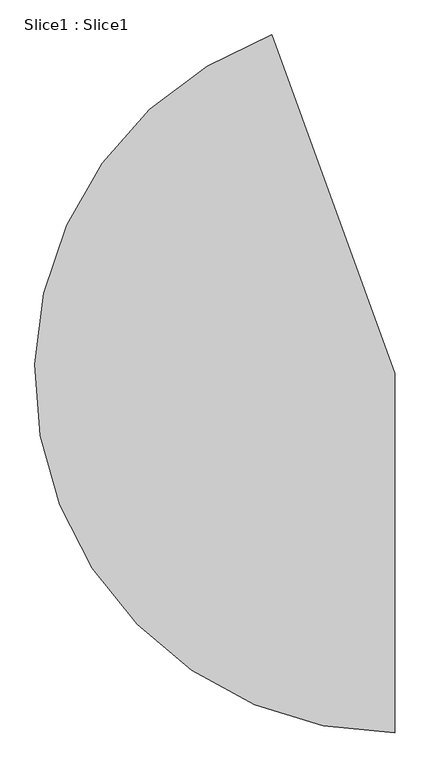
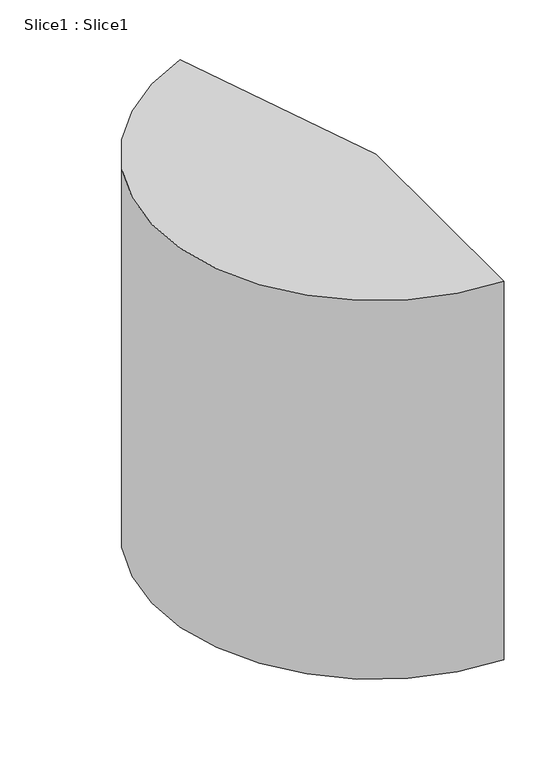
"""IFC4 building model written with IfcOpenShell, lengths in millimetres: proxy geometry, Slice1 : Slice1."""

import ifcopenshell
import ifcopenshell.guid

model = None  # the IFC model being written
_history = None  # IfcOwnerHistory: only IFC2X3 demands one
_inside = {}  # id of a spatial element -> (the spatial element, [elements in it])
_under = {}  # id of a project, library or spatial element -> (it, [spatial elements below it])
_declared = {}  # id of a project -> (the project, [libraries it declares])
_typed = {}  # id of a type object -> (the type object, [elements of that type])
_made_of = {}  # id of a material, layer set ... -> (it, [elements and type objects made of it])


def new_model(schema):
    """Start an empty IFC model of exactly this schema.

    Asked for "IFC4X3", IfcOpenShell would pick the latest addendum, in which some entities
    have other attributes; the version numbers below select the first issue.
    IFC2X3 requires an IfcOwnerHistory on every rooted entity: one is made here for all.
    """
    global model, _history
    if schema == "IFC4X3":
        model = ifcopenshell.file(schema_version=(4, 3, 0, 0))
    else:
        model = ifcopenshell.file(schema=schema)
    _inside.clear()
    _under.clear()
    _declared.clear()
    _typed.clear()
    _made_of.clear()
    _history = None
    if model.schema == "IFC2X3":
        org = make("IfcOrganization", Name="unknown")
        user = make(
            "IfcPersonAndOrganization",
            ThePerson=make("IfcPerson", FamilyName="unknown"),
            TheOrganization=org,
        )
        app = make(
            "IfcApplication",
            ApplicationDeveloper=org,
            Version="unknown",
            ApplicationFullName="unknown",
            ApplicationIdentifier="unknown",
        )
        _history = make(
            "IfcOwnerHistory",
            OwningUser=user,
            OwningApplication=app,
            ChangeAction="ADDED",
            CreationDate=0,
        )
    return model


def make(cls, **values):
    """One entity of the class cls with the attributes given. An attribute that is None is left unset."""
    return model.create_entity(
        cls, **{name: value for name, value in values.items() if value is not None}
    )


def rooted(cls, **values):
    """An entity with a GlobalId (a new one), such as an element, a storey or a relation."""
    return make(cls, GlobalId=ifcopenshell.guid.new(), OwnerHistory=_history, **values)


def si_unit(unit_type, name, prefix=None):
    """IfcSIUnit, for example si_unit("LENGTHUNIT", "METRE", prefix="MILLI")."""
    return make("IfcSIUnit", UnitType=unit_type, Prefix=prefix, Name=name)


def assignment(units):
    """IfcUnitAssignment: the units of a project."""
    return None if units is None else make("IfcUnitAssignment", Units=units)


def point(xyz):
    """IfcCartesianPoint."""
    return None if xyz is None else make("IfcCartesianPoint", Coordinates=xyz)


def direction(xyz):
    """IfcDirection."""
    return None if xyz is None else make("IfcDirection", DirectionRatios=xyz)


def frame(location, z_axis=None, x_axis=None):
    """IfcAxis2Placement3D, a coordinate frame: its origin and axes. An axis left out is left unset."""
    return make(
        "IfcAxis2Placement3D",
        Location=point(location),
        Axis=direction(z_axis),
        RefDirection=direction(x_axis),
    )


def frame_2d(location, x_axis=None):
    """IfcAxis2Placement2D, a coordinate frame in the plane: its origin and x axis."""
    return make(
        "IfcAxis2Placement2D", Location=point(location), RefDirection=direction(x_axis)
    )


def origin():
    """The frame at (0, 0, 0) with its axes left unset."""
    return frame((0.0, 0.0, 0.0))


def origin_with_axes():
    """The frame at (0, 0, 0) with the z axis (0, 0, 1) and the x axis (1, 0, 0) written out."""
    return frame((0.0, 0.0, 0.0), z_axis=(0.0, 0.0, 1.0), x_axis=(1.0, 0.0, 0.0))


def origin_2d():
    """The frame at (0, 0) in the plane with its x axis left unset."""
    return frame_2d((0.0, 0.0))


def place(relative_to, where):
    """IfcLocalPlacement: puts the frame where relative to a parent placement (None: the world)."""
    return make(
        "IfcLocalPlacement", PlacementRelTo=relative_to, RelativePlacement=where
    )


def context(
    kind, dimensions, precision=None, world=None, true_north=None, identifier=None
):
    """IfcGeometricRepresentationContext, for example the 3D "Model" context."""
    return make(
        "IfcGeometricRepresentationContext",
        ContextIdentifier=identifier,
        ContextType=kind,
        CoordinateSpaceDimension=dimensions,
        Precision=precision,
        WorldCoordinateSystem=world,
        TrueNorth=true_north,
    )


def project(units=None, contexts=None):
    """IfcProject with its units and contexts."""
    return rooted(
        "IfcProject",
        Name="project",
        RepresentationContexts=contexts,
        UnitsInContext=assignment(units),
    )


def spatial(cls, under=None, at=None, **own):
    """A site, building, storey or space (cls), placed at a placement, below another one or the project."""
    s = rooted(cls, ObjectPlacement=at, **own)
    if under is not None:
        _under.setdefault(under.id(), (under, []))[1].append(s)
    return s


def polyline(points):
    """IfcPolyline through the points."""
    return make("IfcPolyline", Points=[point(p) for p in points])


def circle_curve(where, radius):
    """IfcCircle in the frame where."""
    return make("IfcCircle", Position=where, Radius=radius)


def trimmed(basis, trim1, trim2, sense, master):
    """IfcTrimmedCurve: the piece of a basis curve between two trims."""
    return make(
        "IfcTrimmedCurve",
        BasisCurve=basis,
        Trim1=trim1,
        Trim2=trim2,
        SenseAgreement=sense,
        MasterRepresentation=master,
    )


def segment(curve, same_sense, transition):
    """IfcCompositeCurveSegment."""
    return make(
        "IfcCompositeCurveSegment",
        Transition=transition,
        SameSense=same_sense,
        ParentCurve=curve,
    )


def composite_curve(segments, self_intersect=None):
    """IfcCompositeCurve: segments joined end to end."""
    return make("IfcCompositeCurve", Segments=segments, SelfIntersect=self_intersect)


def outline(outer, holes=None, kind="AREA"):
    """IfcArbitraryClosedProfileDef: a profile drawn as a closed curve; with holes, ...WithVoids."""
    if holes is None:
        return make("IfcArbitraryClosedProfileDef", ProfileType=kind, OuterCurve=outer)
    return make(
        "IfcArbitraryProfileDefWithVoids",
        ProfileType=kind,
        OuterCurve=outer,
        InnerCurves=holes,
    )


def extrude(swept, where, along, depth):
    """IfcExtrudedAreaSolid: the profile swept, set in the frame where, extruded along a direction by depth."""
    return make(
        "IfcExtrudedAreaSolid",
        SweptArea=swept,
        Position=where,
        ExtrudedDirection=direction(along),
        Depth=depth,
    )


def shape(context_of_items, identifier, shape_type, items):
    """IfcShapeRepresentation: the items that make up one representation, for example the "Body"."""
    return make(
        "IfcShapeRepresentation",
        ContextOfItems=context_of_items,
        RepresentationIdentifier=identifier,
        RepresentationType=shape_type,
        Items=items,
    )


def source(mapping_origin, context_of_items, identifier, shape_type, items):
    """IfcRepresentationMap: a shape defined once, which mapped items show again and again."""
    return make(
        "IfcRepresentationMap",
        MappingOrigin=mapping_origin,
        MappedRepresentation=shape(context_of_items, identifier, shape_type, items),
    )


def transform(
    local_origin,
    x_axis=None,
    y_axis=None,
    z_axis=None,
    scale=None,
    scale2=None,
    scale3=None,
    uniform=True,
):
    """IfcCartesianTransformationOperator3D, or its non-uniform kind. x_axis, y_axis, z_axis: its Axis1, 2, 3."""
    if uniform:
        return make(
            "IfcCartesianTransformationOperator3D",
            Axis1=direction(x_axis),
            Axis2=direction(y_axis),
            LocalOrigin=point(local_origin),
            Scale=scale,
            Axis3=direction(z_axis),
        )
    return make(
        "IfcCartesianTransformationOperator3DnonUniform",
        Axis1=direction(x_axis),
        Axis2=direction(y_axis),
        LocalOrigin=point(local_origin),
        Scale=scale,
        Axis3=direction(z_axis),
        Scale2=scale2,
        Scale3=scale3,
    )


def mapped(mapping_source, mapping_target):
    """IfcMappedItem: shows the shape of a source again, moved by a transform."""
    return make(
        "IfcMappedItem", MappingSource=mapping_source, MappingTarget=mapping_target
    )


def made_of(thing, what):
    """Note that an element or type object is made of a material, layer set ...; save() writes the relation."""
    if what is not None:
        _made_of.setdefault(what.id(), (what, []))[1].append(thing)
    return thing


def element(
    cls,
    number,
    at=None,
    inside=None,
    cuts=None,
    type_object=None,
    material=None,
    context=None,
    identifier="Body",
    shape_type=None,
    held_by="IfcProductDefinitionShape",
    body=None,
    shapes=None,
    **own,
):
    """One element of the class cls, such as IfcWall. Its Tag is "e" and its number.

    at: its placement. inside: the storey or other place that contains it. cuts: it is an
    opening in that element (IfcRelVoidsElement). A single representation is given by context,
    identifier, shape_type and body (its items); several are given by shapes. held_by: the class
    of the entity that holds the representations. save() writes the other relations.
    """
    e = rooted(cls, Tag="e%d" % number, ObjectPlacement=at, **own)
    if body is not None:
        shapes = [shape(context, identifier, shape_type, body)]
    if shapes is not None:
        e.Representation = make(held_by, Representations=shapes)
    if inside is not None:
        _inside.setdefault(inside.id(), (inside, []))[1].append(e)
    if cuts is not None:
        rooted(
            "IfcRelVoidsElement", RelatingBuildingElement=cuts, RelatedOpeningElement=e
        )
    if type_object is not None:
        _typed.setdefault(type_object.id(), (type_object, []))[1].append(e)
    return made_of(e, material)


def aggregate(whole, parts):
    """IfcRelAggregates: a whole, such as a stair, and the parts it consists of."""
    return rooted("IfcRelAggregates", RelatingObject=whole, RelatedObjects=parts)


def save(model, path):
    """Write the relations noted so far, then the file.

    IfcRelAggregates (storeys below a building ...), IfcRelContainedInSpatialStructure (elements
    in a storey), IfcRelDefinesByType, IfcRelAssociatesMaterial and IfcRelDeclares: one each for
    every whole, place, type object, material and project.
    """
    for whole, parts in _under.values():
        aggregate(whole, parts)
    for where, things in _inside.values():
        rooted(
            "IfcRelContainedInSpatialStructure",
            RelatedElements=things,
            RelatingStructure=where,
        )
    for kind, things in _typed.values():
        rooted("IfcRelDefinesByType", RelatedObjects=things, RelatingType=kind)
    for what, things in _made_of.values():
        rooted("IfcRelAssociatesMaterial", RelatedObjects=things, RelatingMaterial=what)
    for by, libraries in _declared.values():
        rooted("IfcRelDeclares", RelatingContext=by, RelatedDefinitions=libraries)
    model.write(path)


def slice1_slice1_33919d9d(model_context):
    return source(origin(), model_context, "Body", "SweptSolid", [
        extrude(outline(composite_curve([segment(trimmed(circle_curve(origin_2d(), 1100.0), [point((0.0, -1100.0))], [point((-376.2221577, 1033.6618829))], False, "CARTESIAN"), True, "CONTINUOUS"), segment(polyline([(-376.2221577, 1033.6618829), (0.0, 0.0), (0.0, -1100.0)]), True, "CONTINUOUS")], self_intersect=False)), origin_with_axes(), (0.0, 0.0, 1.0), 1989.1578093),
    ])


if __name__ == "__main__":
    model = new_model("IFC4")
    model_context = context("Model", 3, world=origin())
    ifc_project = project(units=[si_unit("LENGTHUNIT", "METRE", prefix="MILLI")], contexts=[model_context])
    site = spatial("IfcSite", under=ifc_project)
    building = spatial("IfcBuilding", under=site)
    placement = place(None, origin())
    slice1_slice1_shape = slice1_slice1_33919d9d(model_context)
    element("IfcBuildingElementProxy", 1, Name="Slice1 : Slice1", ObjectType="Slice1 : Slice1", at=placement, inside=building, context=model_context, shape_type="MappedRepresentation", body=[
        mapped(slice1_slice1_shape, transform((0.0, 0.0, 0.0), x_axis=(1.0, 0.0, 0.0), y_axis=(0.0, 1.0, 0.0), z_axis=(0.0, 0.0, 1.0))),
    ])
    save(model, "model.ifc")
